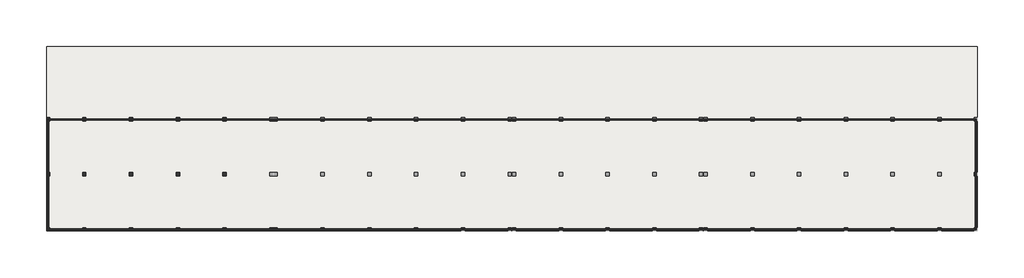
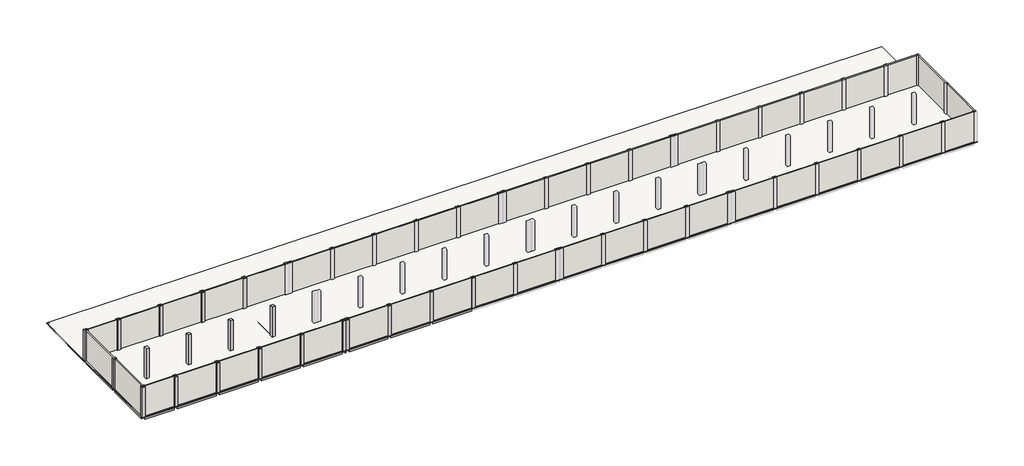
# One storey, part 1 of 4: 38 beams, 20 columns, 4 walls, 2 roofs.
"""IFC4 building model written with IfcOpenShell, lengths in millimetres."""

from ifc_helpers import new_model, si_unit, frame, origin, place, context, project, spatial, polyline, outline, extrude, faceted_brep, element, save

model = new_model("IFC4")

# Units and contexts
model_context = context("Model", 3, world=origin())
ifc_project = project(units=[si_unit("LENGTHUNIT", "METRE", prefix="MILLI")], contexts=[model_context])

# Site, building, storey
site = spatial("IfcSite", under=ifc_project)
building = spatial("IfcBuilding", under=site)
storey = spatial("IfcBuildingStorey", under=building, Name="03_T.O.C_1", Elevation=6949.9618634)

# Beams
placement = place(None, origin())
element("IfcBeam", 1, ObjectType="RC Beam_Rectangular : H_SB_AR_S16_B300xH600", at=placement, inside=storey, context=model_context, shape_type="SweptSolid", body=[
    extrude(outline(polyline([(-4070.0, -6150.4791411), (-4070.0, -5850.4791411), (1630.0, -5850.4791411), (1630.0, -6150.4791411), (-4070.0, -6150.4791411)])), frame((0.0, 0.0, 6349.9618634), z_axis=(0.0, 0.0, 1.0), x_axis=(1.0, 0.0, 0.0)), (0.0, 0.0, 1.0), 499.0),
])
element("IfcBeam", 2, ObjectType="RC Beam_Rectangular : H_SB_AR_S16_B300xH600", at=placement, inside=storey, context=model_context, shape_type="SweptSolid", body=[
    extrude(outline(polyline([(2230.0, -6150.4791411), (2230.0, -5850.4791411), (9830.0, -5850.4791411), (9830.0, -6150.4791411), (2230.0, -6150.4791411)])), frame((0.0, 0.0, 6349.9618634), z_axis=(0.0, 0.0, 1.0), x_axis=(1.0, 0.0, 0.0)), (0.0, 0.0, 1.0), 499.0),
])
element("IfcBeam", 3, ObjectType="RC Beam_Rectangular : H_SB_AR_S16_B300xH600", at=placement, inside=storey, context=model_context, shape_type="SweptSolid", body=[
    extrude(outline(polyline([(10430.0, -6150.4791411), (10430.0, -5850.4791411), (18030.0, -5850.4791411), (18030.0, -6150.4791411), (10430.0, -6150.4791411)])), frame((0.0, 0.0, 6349.9618634), z_axis=(0.0, 0.0, 1.0), x_axis=(1.0, 0.0, 0.0)), (0.0, 0.0, 1.0), 499.0),
])
element("IfcBeam", 4, ObjectType="RC Beam_Rectangular : H_SB_AR_S16_B300xH600", at=placement, inside=storey, context=model_context, shape_type="SweptSolid", body=[
    extrude(outline(polyline([(18630.0, -6150.4791411), (18630.0, -5850.4791411), (26230.0, -5850.4791411), (26230.0, -6150.4791411), (18630.0, -6150.4791411)])), frame((0.0, 0.0, 6349.9618634), z_axis=(0.0, 0.0, 1.0), x_axis=(1.0, 0.0, 0.0)), (0.0, 0.0, 1.0), 499.0),
])
element("IfcBeam", 5, ObjectType="RC Beam_Rectangular : H_SB_AR_S16_B300xH600", at=placement, inside=storey, context=model_context, shape_type="SweptSolid", body=[
    extrude(outline(polyline([(26830.0, -6150.4791411), (26830.0, -5850.4791411), (34430.0, -5850.4791411), (34430.0, -6150.4791411), (26830.0, -6150.4791411)])), frame((0.0, 0.0, 6349.9618634), z_axis=(0.0, 0.0, 1.0), x_axis=(1.0, 0.0, 0.0)), (0.0, 0.0, 1.0), 499.0),
])
element("IfcBeam", 6, ObjectType="RC Beam_Rectangular : H_SB_AR_S16_B300xH600", at=placement, inside=storey, context=model_context, shape_type="SweptSolid", body=[
    extrude(outline(polyline([(-4070.0, -15800.4791411), (-4070.0, -15500.4791411), (1630.0, -15500.4791411), (1630.0, -15800.4791411), (-4070.0, -15800.4791411)])), frame((0.0, 0.0, 6349.9618634), z_axis=(0.0, 0.0, 1.0), x_axis=(1.0, 0.0, 0.0)), (0.0, 0.0, 1.0), 499.0),
])
element("IfcBeam", 7, ObjectType="RC Beam_Rectangular : H_SB_AR_S16_B300xH600", at=placement, inside=storey, context=model_context, shape_type="SweptSolid", body=[
    extrude(outline(polyline([(2230.0, -15800.4791411), (2230.0, -15500.4791411), (9830.0, -15500.4791411), (9830.0, -15800.4791411), (2230.0, -15800.4791411)])), frame((0.0, 0.0, 6349.9618634), z_axis=(0.0, 0.0, 1.0), x_axis=(1.0, 0.0, 0.0)), (0.0, 0.0, 1.0), 499.0),
])
element("IfcBeam", 8, ObjectType="RC Beam_Rectangular : H_SB_AR_S16_B300xH600", at=placement, inside=storey, context=model_context, shape_type="SweptSolid", body=[
    extrude(outline(polyline([(10430.0, -15800.4791411), (10430.0, -15500.4791411), (18030.0, -15500.4791411), (18030.0, -15800.4791411), (10430.0, -15800.4791411)])), frame((0.0, 0.0, 6349.9618634), z_axis=(0.0, 0.0, 1.0), x_axis=(1.0, 0.0, 0.0)), (0.0, 0.0, 1.0), 499.0),
])
element("IfcBeam", 9, ObjectType="RC Beam_Rectangular : H_SB_AR_S16_B300xH600", at=placement, inside=storey, context=model_context, shape_type="SweptSolid", body=[
    extrude(outline(polyline([(18630.0, -15800.4791411), (18630.0, -15500.4791411), (26230.0, -15500.4791411), (26230.0, -15800.4791411), (18630.0, -15800.4791411)])), frame((0.0, 0.0, 6349.9618634), z_axis=(0.0, 0.0, 1.0), x_axis=(1.0, 0.0, 0.0)), (0.0, 0.0, 1.0), 499.0),
])
element("IfcBeam", 10, ObjectType="RC Beam_Rectangular : H_SB_AR_S16_B300xH600", at=placement, inside=storey, context=model_context, shape_type="SweptSolid", body=[
    extrude(outline(polyline([(26830.0, -15800.4791411), (26830.0, -15500.4791411), (34430.0, -15500.4791411), (34430.0, -15800.4791411), (26830.0, -15800.4791411)])), frame((0.0, 0.0, 6349.9618634), z_axis=(0.0, 0.0, 1.0), x_axis=(1.0, 0.0, 0.0)), (0.0, 0.0, 1.0), 499.0),
])
element("IfcBeam", 11, ObjectType="RC Beam_Rectangular : H_SB_AR_S16_B300xH600", at=placement, inside=storey, context=model_context, shape_type="SweptSolid", body=[
    extrude(outline(polyline([(-4070.0, -25450.4791411), (-4070.0, -25150.4791411), (1630.0, -25150.4791411), (1630.0, -25450.4791411), (-4070.0, -25450.4791411)])), frame((0.0, 0.0, 6349.9618634), z_axis=(0.0, 0.0, 1.0), x_axis=(1.0, 0.0, 0.0)), (0.0, 0.0, 1.0), 499.0),
])
element("IfcBeam", 12, ObjectType="RC Beam_Rectangular : H_SB_AR_S16_B300xH600", at=placement, inside=storey, context=model_context, shape_type="SweptSolid", body=[
    extrude(outline(polyline([(2230.0, -25450.4791411), (2230.0, -25150.4791411), (9830.0, -25150.4791411), (9830.0, -25450.4791411), (2230.0, -25450.4791411)])), frame((0.0, 0.0, 6349.9618634), z_axis=(0.0, 0.0, 1.0), x_axis=(1.0, 0.0, 0.0)), (0.0, 0.0, 1.0), 499.0),
])
element("IfcBeam", 13, ObjectType="RC Beam_Rectangular : H_SB_AR_S16_B300xH600", at=placement, inside=storey, context=model_context, shape_type="SweptSolid", body=[
    extrude(outline(polyline([(10430.0, -25450.4791411), (10430.0, -25150.4791411), (18030.0, -25150.4791411), (18030.0, -25450.4791411), (10430.0, -25450.4791411)])), frame((0.0, 0.0, 6349.9618634), z_axis=(0.0, 0.0, 1.0), x_axis=(1.0, 0.0, 0.0)), (0.0, 0.0, 1.0), 499.0),
])
element("IfcBeam", 14, ObjectType="RC Beam_Rectangular : H_SB_AR_S16_B300xH600", at=placement, inside=storey, context=model_context, shape_type="SweptSolid", body=[
    extrude(outline(polyline([(18630.0, -25450.4791411), (18630.0, -25150.4791411), (26230.0, -25150.4791411), (26230.0, -25450.4791411), (18630.0, -25450.4791411)])), frame((0.0, 0.0, 6349.9618634), z_axis=(0.0, 0.0, 1.0), x_axis=(1.0, 0.0, 0.0)), (0.0, 0.0, 1.0), 499.0),
])
element("IfcBeam", 15, ObjectType="RC Beam_Rectangular : H_SB_AR_S16_B300xH600", at=placement, inside=storey, context=model_context, shape_type="SweptSolid", body=[
    extrude(outline(polyline([(26830.0, -25450.4791411), (26830.0, -25150.4791411), (34430.0, -25150.4791411), (34430.0, -25450.4791411), (26830.0, -25450.4791411)])), frame((0.0, 0.0, 6349.9618634), z_axis=(0.0, 0.0, 1.0), x_axis=(1.0, 0.0, 0.0)), (0.0, 0.0, 1.0), 499.0),
])
element("IfcBeam", 16, ObjectType="RC Beam_Rectangular : H_SB_AR_S16_B300xH600", at=placement, inside=storey, context=model_context, shape_type="SweptSolid", body=[
    extrude(outline(polyline([(35030.0, -25450.4791411), (35030.0, -25150.4791411), (35180.0, -25150.4791411), (35180.0, -25450.4791411), (35030.0, -25450.4791411)])), frame((0.0, 0.0, 6349.9618634), z_axis=(0.0, 0.0, 1.0), x_axis=(1.0, 0.0, 0.0)), (0.0, 0.0, 1.0), 499.0),
])
element("IfcBeam", 17, ObjectType="RC Beam_Rectangular : H_SB_AR_S16_B300xH600", at=placement, inside=storey, context=model_context, shape_type="SweptSolid", body=[
    extrude(outline(polyline([(35780.0, -25450.4791411), (35780.0, -25150.4791411), (43380.0, -25150.4791411), (43380.0, -25450.4791411), (35780.0, -25450.4791411)])), frame((0.0, 0.0, 6349.9618634), z_axis=(0.0, 0.0, 1.0), x_axis=(1.0, 0.0, 0.0)), (0.0, 0.0, 1.0), 499.0),
])
element("IfcBeam", 18, ObjectType="RC Beam_Rectangular : H_SB_AR_S16_B300xH600", at=placement, inside=storey, context=model_context, shape_type="SweptSolid", body=[
    extrude(outline(polyline([(43980.0, -25450.4791411), (43980.0, -25150.4791411), (51580.0, -25150.4791411), (51580.0, -25450.4791411), (43980.0, -25450.4791411)])), frame((0.0, 0.0, 6349.9618634), z_axis=(0.0, 0.0, 1.0), x_axis=(1.0, 0.0, 0.0)), (0.0, 0.0, 1.0), 499.0),
])
element("IfcBeam", 19, ObjectType="RC Beam_Rectangular : H_SB_AR_S16_B300xH600", at=placement, inside=storey, context=model_context, shape_type="SweptSolid", body=[
    extrude(outline(polyline([(52180.0, -25450.4791411), (52180.0, -25150.4791411), (59780.0, -25150.4791411), (59780.0, -25450.4791411), (52180.0, -25450.4791411)])), frame((0.0, 0.0, 6349.9618634), z_axis=(0.0, 0.0, 1.0), x_axis=(1.0, 0.0, 0.0)), (0.0, 0.0, 1.0), 499.0),
])
element("IfcBeam", 20, ObjectType="RC Beam_Rectangular : H_SB_AR_S16_B300xH600", at=placement, inside=storey, context=model_context, shape_type="SweptSolid", body=[
    extrude(outline(polyline([(-4520.0, -15950.4791411), (-4220.0, -15950.4791411), (-4220.0, -25000.4791411), (-4520.0, -25000.4791411), (-4520.0, -15950.4791411)])), frame((0.0, 0.0, 6349.9618634), z_axis=(0.0, 0.0, 1.0), x_axis=(1.0, 0.0, 0.0)), (0.0, 0.0, 1.0), 499.0),
])
element("IfcBeam", 21, ObjectType="RC Beam_Rectangular : H_SB_AR_S16_B300xH600", at=placement, inside=storey, context=model_context, shape_type="SweptSolid", body=[
    extrude(outline(polyline([(-4520.0, -6300.4791411), (-4220.0, -6300.4791411), (-4220.0, -15350.4791411), (-4520.0, -15350.4791411), (-4520.0, -6300.4791411)])), frame((0.0, 0.0, 6349.9618634), z_axis=(0.0, 0.0, 1.0), x_axis=(1.0, 0.0, 0.0)), (0.0, 0.0, 1.0), 499.0),
])
element("IfcBeam", 22, ObjectType="RC Beam_Rectangular : H_SB_AR_S16_B300xH600", at=placement, inside=storey, context=model_context, shape_type="SweptSolid", body=[
    extrude(outline(polyline([(-4520.0, -50.4791411), (-4220.0, -50.4791411), (-4220.0, -5700.4791411), (-4520.0, -5700.4791411), (-4520.0, -50.4791411)])), frame((0.0, 0.0, 6349.9618634), z_axis=(0.0, 0.0, 1.0), x_axis=(1.0, 0.0, 0.0)), (0.0, 0.0, 1.0), 499.0),
])
element("IfcBeam", 23, ObjectType="RC Beam_Rectangular : H_SB_AR_S16_B300xH600", at=placement, inside=storey, context=model_context, shape_type="SweptSolid", body=[
    extrude(outline(polyline([(1780.0, -15950.4791411), (2080.0, -15950.4791411), (2080.0, -25000.4791411), (1780.0, -25000.4791411), (1780.0, -15950.4791411)])), frame((0.0, 0.0, 6349.9618634), z_axis=(0.0, 0.0, 1.0), x_axis=(1.0, 0.0, 0.0)), (0.0, 0.0, 1.0), 499.0),
])
element("IfcBeam", 24, ObjectType="RC Beam_Rectangular : H_SB_AR_S16_B300xH600", at=placement, inside=storey, context=model_context, shape_type="SweptSolid", body=[
    extrude(outline(polyline([(1780.0, -6300.4791411), (2080.0, -6300.4791411), (2080.0, -15350.4791411), (1780.0, -15350.4791411), (1780.0, -6300.4791411)])), frame((0.0, 0.0, 6349.9618634), z_axis=(0.0, 0.0, 1.0), x_axis=(1.0, 0.0, 0.0)), (0.0, 0.0, 1.0), 499.0),
])
element("IfcBeam", 25, ObjectType="RC Beam_Rectangular : H_SB_AR_S16_B300xH600", at=placement, inside=storey, context=model_context, shape_type="SweptSolid", body=[
    extrude(outline(polyline([(1780.0, 99.5208589), (2080.0, 99.5208589), (2080.0, -5700.4791411), (1780.0, -5700.4791411), (1780.0, 99.5208589)])), frame((0.0, 0.0, 6349.9618634), z_axis=(0.0, 0.0, 1.0), x_axis=(1.0, 0.0, 0.0)), (0.0, 0.0, 1.0), 499.0),
])
element("IfcBeam", 26, ObjectType="RC Beam_Rectangular : H_SB_AR_S16_B300xH600", at=placement, inside=storey, context=model_context, shape_type="SweptSolid", body=[
    extrude(outline(polyline([(9980.0, -15950.4791411), (10280.0, -15950.4791411), (10280.0, -25000.4791411), (9980.0, -25000.4791411), (9980.0, -15950.4791411)])), frame((0.0, 0.0, 6349.9618634), z_axis=(0.0, 0.0, 1.0), x_axis=(1.0, 0.0, 0.0)), (0.0, 0.0, 1.0), 499.0),
])
element("IfcBeam", 27, ObjectType="RC Beam_Rectangular : H_SB_AR_S16_B300xH600", at=placement, inside=storey, context=model_context, shape_type="SweptSolid", body=[
    extrude(outline(polyline([(9980.0, -6300.4791411), (10280.0, -6300.4791411), (10280.0, -15350.4791411), (9980.0, -15350.4791411), (9980.0, -6300.4791411)])), frame((0.0, 0.0, 6349.9618634), z_axis=(0.0, 0.0, 1.0), x_axis=(1.0, 0.0, 0.0)), (0.0, 0.0, 1.0), 499.0),
])
element("IfcBeam", 28, ObjectType="RC Beam_Rectangular : H_SB_AR_S16_B300xH600", at=placement, inside=storey, context=model_context, shape_type="SweptSolid", body=[
    extrude(outline(polyline([(9980.0, 99.5208589), (10280.0, 99.5208589), (10280.0, -5700.4791411), (9980.0, -5700.4791411), (9980.0, 99.5208589)])), frame((0.0, 0.0, 6349.9618634), z_axis=(0.0, 0.0, 1.0), x_axis=(1.0, 0.0, 0.0)), (0.0, 0.0, 1.0), 499.0),
])
element("IfcBeam", 29, ObjectType="RC Beam_Rectangular : H_SB_AR_S16_B300xH600", at=placement, inside=storey, context=model_context, shape_type="SweptSolid", body=[
    extrude(outline(polyline([(18180.0, -15950.4791411), (18480.0, -15950.4791411), (18480.0, -25000.4791411), (18180.0, -25000.4791411), (18180.0, -15950.4791411)])), frame((0.0, 0.0, 6349.9618634), z_axis=(0.0, 0.0, 1.0), x_axis=(1.0, 0.0, 0.0)), (0.0, 0.0, 1.0), 499.0),
])
element("IfcBeam", 30, ObjectType="RC Beam_Rectangular : H_SB_AR_S16_B300xH600", at=placement, inside=storey, context=model_context, shape_type="SweptSolid", body=[
    extrude(outline(polyline([(18180.0, -6300.4791411), (18480.0, -6300.4791411), (18480.0, -15350.4791411), (18180.0, -15350.4791411), (18180.0, -6300.4791411)])), frame((0.0, 0.0, 6349.9618634), z_axis=(0.0, 0.0, 1.0), x_axis=(1.0, 0.0, 0.0)), (0.0, 0.0, 1.0), 499.0),
])
element("IfcBeam", 31, ObjectType="RC Beam_Rectangular : H_SB_AR_S16_B300xH600", at=placement, inside=storey, context=model_context, shape_type="SweptSolid", body=[
    extrude(outline(polyline([(18180.0, 99.5208589), (18480.0, 99.5208589), (18480.0, -5700.4791411), (18180.0, -5700.4791411), (18180.0, 99.5208589)])), frame((0.0, 0.0, 6349.9618634), z_axis=(0.0, 0.0, 1.0), x_axis=(1.0, 0.0, 0.0)), (0.0, 0.0, 1.0), 499.0),
])
element("IfcBeam", 32, ObjectType="RC Beam_Rectangular : H_SB_AR_S16_B300xH600", at=placement, inside=storey, context=model_context, shape_type="SweptSolid", body=[
    extrude(outline(polyline([(26380.0, -15950.4791411), (26680.0, -15950.4791411), (26680.0, -25000.4791411), (26380.0, -25000.4791411), (26380.0, -15950.4791411)])), frame((0.0, 0.0, 6349.9618634), z_axis=(0.0, 0.0, 1.0), x_axis=(1.0, 0.0, 0.0)), (0.0, 0.0, 1.0), 499.0),
])
element("IfcBeam", 33, ObjectType="RC Beam_Rectangular : H_SB_AR_S16_B300xH600", at=placement, inside=storey, context=model_context, shape_type="SweptSolid", body=[
    extrude(outline(polyline([(26380.0, -6300.4791411), (26680.0, -6300.4791411), (26680.0, -15350.4791411), (26380.0, -15350.4791411), (26380.0, -6300.4791411)])), frame((0.0, 0.0, 6349.9618634), z_axis=(0.0, 0.0, 1.0), x_axis=(1.0, 0.0, 0.0)), (0.0, 0.0, 1.0), 499.0),
])
element("IfcBeam", 34, ObjectType="RC Beam_Rectangular : H_SB_AR_S16_B300xH600", at=placement, inside=storey, context=model_context, shape_type="SweptSolid", body=[
    extrude(outline(polyline([(26380.0, 99.5208589), (26680.0, 99.5208589), (26680.0, -5700.4791411), (26380.0, -5700.4791411), (26380.0, 99.5208589)])), frame((0.0, 0.0, 6349.9618634), z_axis=(0.0, 0.0, 1.0), x_axis=(1.0, 0.0, 0.0)), (0.0, 0.0, 1.0), 499.0),
])
element("IfcBeam", 35, ObjectType="RC Beam_Rectangular : H_SB_AR_S16_B300xH600", at=placement, inside=storey, context=model_context, shape_type="SweptSolid", body=[
    extrude(outline(polyline([(34580.0, -15950.4791411), (34880.0, -15950.4791411), (34880.0, -25000.4791411), (34580.0, -25000.4791411), (34580.0, -15950.4791411)])), frame((0.0, 0.0, 6349.9618634), z_axis=(0.0, 0.0, 1.0), x_axis=(1.0, 0.0, 0.0)), (0.0, 0.0, 1.0), 499.0),
])
element("IfcBeam", 36, ObjectType="RC Beam_Rectangular : H_SB_AR_S16_B300xH600", at=placement, inside=storey, context=model_context, shape_type="SweptSolid", body=[
    extrude(outline(polyline([(35330.0, -15950.4791411), (35630.0, -15950.4791411), (35630.0, -25000.4791411), (35330.0, -25000.4791411), (35330.0, -15950.4791411)])), frame((0.0, 0.0, 6349.9618634), z_axis=(0.0, 0.0, 1.0), x_axis=(1.0, 0.0, 0.0)), (0.0, 0.0, 1.0), 499.0),
])
element("IfcBeam", 37, ObjectType="RC Beam_Rectangular : H_SB_AR_S16_B300xH600", at=placement, inside=storey, context=model_context, shape_type="SweptSolid", body=[
    extrude(outline(polyline([(43530.0, -15950.4791411), (43830.0, -15950.4791411), (43830.0, -25000.4791411), (43530.0, -25000.4791411), (43530.0, -15950.4791411)])), frame((0.0, 0.0, 6349.9618634), z_axis=(0.0, 0.0, 1.0), x_axis=(1.0, 0.0, 0.0)), (0.0, 0.0, 1.0), 499.0),
])
element("IfcBeam", 38, ObjectType="RC Beam_Rectangular : H_SB_AR_S16_B300xH600", at=placement, inside=storey, context=model_context, shape_type="SweptSolid", body=[
    extrude(outline(polyline([(51730.0, -15950.4791411), (52030.0, -15950.4791411), (52030.0, -25000.4791411), (51730.0, -25000.4791411), (51730.0, -15950.4791411)])), frame((0.0, 0.0, 6349.9618634), z_axis=(0.0, 0.0, 1.0), x_axis=(1.0, 0.0, 0.0)), (0.0, 0.0, 1.0), 499.0),
])

# Columns
element("IfcColumn", 39, ObjectType="RC_Column_Rectangular : H_SC_AR_S15_W600xL600", at=placement, inside=storey, context=model_context, shape_type="SweptSolid", body=[
    extrude(outline(polyline([(-4070.0, -5700.4791411), (-4070.0, -6300.4791411), (-4670.0, -6300.4791411), (-4670.0, -5700.4791411), (-4070.0, -5700.4791411)])), frame((0.0, 0.0, 6949.9618634), z_axis=(0.0, 0.0, 1.0), x_axis=(1.0, 0.0, 0.0)), (0.0, 0.0, 1.0), 6200.0),
])
element("IfcColumn", 40, ObjectType="RC_Column_Rectangular : H_SC_AR_S15_W600xL600", at=placement, inside=storey, context=model_context, shape_type="SweptSolid", body=[
    extrude(outline(polyline([(2230.0, -5700.4791411), (2230.0, -6300.4791411), (1630.0, -6300.4791411), (1630.0, -5700.4791411), (2230.0, -5700.4791411)])), frame((0.0, 0.0, 6949.9618634), z_axis=(0.0, 0.0, 1.0), x_axis=(1.0, 0.0, 0.0)), (0.0, 0.0, 1.0), 6200.0),
])
element("IfcColumn", 41, ObjectType="RC_Column_Rectangular : H_SC_AR_S15_W600xL600", at=placement, inside=storey, context=model_context, shape_type="SweptSolid", body=[
    extrude(outline(polyline([(10430.0, -5700.4791411), (10430.0, -6300.4791411), (9830.0, -6300.4791411), (9830.0, -5700.4791411), (10430.0, -5700.4791411)])), frame((0.0, 0.0, 6949.9618634), z_axis=(0.0, 0.0, 1.0), x_axis=(1.0, 0.0, 0.0)), (0.0, 0.0, 1.0), 6200.0),
])
element("IfcColumn", 42, ObjectType="RC_Column_Rectangular : H_SC_AR_S15_W600xL600", at=placement, inside=storey, context=model_context, shape_type="SweptSolid", body=[
    extrude(outline(polyline([(18630.0, -5700.4791411), (18630.0, -6300.4791411), (18030.0, -6300.4791411), (18030.0, -5700.4791411), (18630.0, -5700.4791411)])), frame((0.0, 0.0, 6949.9618634), z_axis=(0.0, 0.0, 1.0), x_axis=(1.0, 0.0, 0.0)), (0.0, 0.0, 1.0), 6200.0),
])
element("IfcColumn", 43, ObjectType="RC_Column_Rectangular : H_SC_AR_S15_W600xL600", at=placement, inside=storey, context=model_context, shape_type="SweptSolid", body=[
    extrude(outline(polyline([(26830.0, -5700.4791411), (26830.0, -6300.4791411), (26230.0, -6300.4791411), (26230.0, -5700.4791411), (26830.0, -5700.4791411)])), frame((0.0, 0.0, 6949.9618634), z_axis=(0.0, 0.0, 1.0), x_axis=(1.0, 0.0, 0.0)), (0.0, 0.0, 1.0), 6200.0),
])
element("IfcColumn", 44, ObjectType="RC_Column_Rectangular : H_SC_AR_S15_W600xL600", at=placement, inside=storey, context=model_context, shape_type="SweptSolid", body=[
    extrude(outline(polyline([(-4070.0, -15350.4791411), (-4070.0, -15950.4791411), (-4670.0, -15950.4791411), (-4670.0, -15350.4791411), (-4070.0, -15350.4791411)])), frame((0.0, 0.0, 6949.9618634), z_axis=(0.0, 0.0, 1.0), x_axis=(1.0, 0.0, 0.0)), (0.0, 0.0, 1.0), 6200.0),
])
element("IfcColumn", 45, ObjectType="RC_Column_Rectangular : H_SC_AR_S15_W600xL600", at=placement, inside=storey, context=model_context, shape_type="SweptSolid", body=[
    extrude(outline(polyline([(2230.0, -15350.4791411), (2230.0, -15950.4791411), (1630.0, -15950.4791411), (1630.0, -15350.4791411), (2230.0, -15350.4791411)])), frame((0.0, 0.0, 6949.9618634), z_axis=(0.0, 0.0, 1.0), x_axis=(1.0, 0.0, 0.0)), (0.0, 0.0, 1.0), 6200.0),
])
element("IfcColumn", 46, ObjectType="RC_Column_Rectangular : H_SC_AR_S15_W600xL600", at=placement, inside=storey, context=model_context, shape_type="SweptSolid", body=[
    extrude(outline(polyline([(10430.0, -15350.4791411), (10430.0, -15950.4791411), (9830.0, -15950.4791411), (9830.0, -15350.4791411), (10430.0, -15350.4791411)])), frame((0.0, 0.0, 6949.9618634), z_axis=(0.0, 0.0, 1.0), x_axis=(1.0, 0.0, 0.0)), (0.0, 0.0, 1.0), 6200.0),
])
element("IfcColumn", 47, ObjectType="RC_Column_Rectangular : H_SC_AR_S15_W600xL600", at=placement, inside=storey, context=model_context, shape_type="SweptSolid", body=[
    extrude(outline(polyline([(18630.0, -15350.4791411), (18630.0, -15950.4791411), (18030.0, -15950.4791411), (18030.0, -15350.4791411), (18630.0, -15350.4791411)])), frame((0.0, 0.0, 6949.9618634), z_axis=(0.0, 0.0, 1.0), x_axis=(1.0, 0.0, 0.0)), (0.0, 0.0, 1.0), 6200.0),
])
element("IfcColumn", 48, ObjectType="RC_Column_Rectangular : H_SC_AR_S15_W600xL600", at=placement, inside=storey, context=model_context, shape_type="SweptSolid", body=[
    extrude(outline(polyline([(26830.0, -15350.4791411), (26830.0, -15950.4791411), (26230.0, -15950.4791411), (26230.0, -15350.4791411), (26830.0, -15350.4791411)])), frame((0.0, 0.0, 6949.9618634), z_axis=(0.0, 0.0, 1.0), x_axis=(1.0, 0.0, 0.0)), (0.0, 0.0, 1.0), 6200.0),
])
element("IfcColumn", 49, ObjectType="RC_Column_Rectangular : H_SC_AR_S15_W600xL600", at=placement, inside=storey, context=model_context, shape_type="SweptSolid", body=[
    extrude(outline(polyline([(-4070.0, -25000.4791411), (-4070.0, -25600.4791411), (-4670.0, -25600.4791411), (-4670.0, -25000.4791411), (-4070.0, -25000.4791411)])), frame((0.0, 0.0, 6949.9618634), z_axis=(0.0, 0.0, 1.0), x_axis=(1.0, 0.0, 0.0)), (0.0, 0.0, 1.0), 6200.0),
])
element("IfcColumn", 50, ObjectType="RC_Column_Rectangular : H_SC_AR_S15_W600xL600", at=placement, inside=storey, context=model_context, shape_type="SweptSolid", body=[
    extrude(outline(polyline([(2230.0, -25000.4791411), (2230.0, -25600.4791411), (1630.0, -25600.4791411), (1630.0, -25000.4791411), (2230.0, -25000.4791411)])), frame((0.0, 0.0, 6949.9618634), z_axis=(0.0, 0.0, 1.0), x_axis=(1.0, 0.0, 0.0)), (0.0, 0.0, 1.0), 6200.0),
])
element("IfcColumn", 51, ObjectType="RC_Column_Rectangular : H_SC_AR_S15_W600xL600", at=placement, inside=storey, context=model_context, shape_type="SweptSolid", body=[
    extrude(outline(polyline([(10430.0, -25000.4791411), (10430.0, -25600.4791411), (9830.0, -25600.4791411), (9830.0, -25000.4791411), (10430.0, -25000.4791411)])), frame((0.0, 0.0, 6949.9618634), z_axis=(0.0, 0.0, 1.0), x_axis=(1.0, 0.0, 0.0)), (0.0, 0.0, 1.0), 6200.0),
])
element("IfcColumn", 52, ObjectType="RC_Column_Rectangular : H_SC_AR_S15_W600xL600", at=placement, inside=storey, context=model_context, shape_type="SweptSolid", body=[
    extrude(outline(polyline([(18630.0, -25000.4791411), (18630.0, -25600.4791411), (18030.0, -25600.4791411), (18030.0, -25000.4791411), (18630.0, -25000.4791411)])), frame((0.0, 0.0, 6949.9618634), z_axis=(0.0, 0.0, 1.0), x_axis=(1.0, 0.0, 0.0)), (0.0, 0.0, 1.0), 6200.0),
])
element("IfcColumn", 53, ObjectType="RC_Column_Rectangular : H_SC_AR_S15_W600xL600", at=placement, inside=storey, context=model_context, shape_type="SweptSolid", body=[
    extrude(outline(polyline([(26830.0, -25000.4791411), (26830.0, -25600.4791411), (26230.0, -25600.4791411), (26230.0, -25000.4791411), (26830.0, -25000.4791411)])), frame((0.0, 0.0, 6949.9618634), z_axis=(0.0, 0.0, 1.0), x_axis=(1.0, 0.0, 0.0)), (0.0, 0.0, 1.0), 6200.0),
])
element("IfcColumn", 54, ObjectType="RC_Column_Rectangular : H_SC_AR_S15_W600xL600", at=placement, inside=storey, context=model_context, shape_type="SweptSolid", body=[
    extrude(outline(polyline([(35030.0, -25000.4791411), (35030.0, -25600.4791411), (34430.0, -25600.4791411), (34430.0, -25000.4791411), (35030.0, -25000.4791411)])), frame((0.0, 0.0, 6949.9618634), z_axis=(0.0, 0.0, 1.0), x_axis=(1.0, 0.0, 0.0)), (0.0, 0.0, 1.0), 6200.0),
])
element("IfcColumn", 55, ObjectType="RC_Column_Rectangular : H_SC_AR_S15_W600xL600", at=placement, inside=storey, context=model_context, shape_type="SweptSolid", body=[
    extrude(outline(polyline([(35780.0, -25000.4791411), (35780.0, -25600.4791411), (35180.0, -25600.4791411), (35180.0, -25000.4791411), (35780.0, -25000.4791411)])), frame((0.0, 0.0, 6949.9618634), z_axis=(0.0, 0.0, 1.0), x_axis=(1.0, 0.0, 0.0)), (0.0, 0.0, 1.0), 6200.0),
])
element("IfcColumn", 56, ObjectType="RC_Column_Rectangular : H_SC_AR_S15_W600xL600", at=placement, inside=storey, context=model_context, shape_type="SweptSolid", body=[
    extrude(outline(polyline([(43980.0, -25000.4791411), (43980.0, -25600.4791411), (43380.0, -25600.4791411), (43380.0, -25000.4791411), (43980.0, -25000.4791411)])), frame((0.0, 0.0, 6949.9618634), z_axis=(0.0, 0.0, 1.0), x_axis=(1.0, 0.0, 0.0)), (0.0, 0.0, 1.0), 6200.0),
])
element("IfcColumn", 57, ObjectType="RC_Column_Rectangular : H_SC_AR_S15_W600xL600", at=placement, inside=storey, context=model_context, shape_type="SweptSolid", body=[
    extrude(outline(polyline([(52180.0, -25000.4791411), (52180.0, -25600.4791411), (51580.0, -25600.4791411), (51580.0, -25000.4791411), (52180.0, -25000.4791411)])), frame((0.0, 0.0, 6949.9618634), z_axis=(0.0, 0.0, 1.0), x_axis=(1.0, 0.0, 0.0)), (0.0, 0.0, 1.0), 6200.0),
])
element("IfcColumn", 58, ObjectType="RC_Column_Rectangular : H_SC_AR_S15_W600xL600", at=placement, inside=storey, context=model_context, shape_type="SweptSolid", body=[
    extrude(outline(polyline([(60380.0, -25000.4791411), (60380.0, -25600.4791411), (59780.0, -25600.4791411), (59780.0, -25000.4791411), (60380.0, -25000.4791411)])), frame((0.0, 0.0, 6949.9618634), z_axis=(0.0, 0.0, 1.0), x_axis=(1.0, 0.0, 0.0)), (0.0, 0.0, 1.0), 6200.0),
])

# Roofs
element("IfcRoof", 59, ObjectType="H_RF_AR_B06_Memb_XPS_PE_Protective Conc", at=placement, inside=storey, context=model_context, shape_type="Brep", body=[
    faceted_brep([(158430.0, 6799.5208589, 6848.9618634), (158430.0, 6199.5208589, 6848.9618634), (158430.0, 549.5208589, 6848.9618634), (158430.0, -50.4791411, 6848.9618634), (158430.0, -5700.4791411, 6848.9618634), (158430.0, -6300.4791411, 6848.9618634), (158430.0, -15350.4791411, 6848.9618634), (158430.0, -15950.4791411, 6848.9618634), (158430.0, -25000.4791411, 6848.9618634), (158430.0, -25600.4791411, 6848.9618634), (157830.0, -25600.4791411, 6848.9618634), (152080.0, -25600.4791411, 6848.9618634), (151480.0, -25600.4791411, 6848.9618634), (143880.0, -25600.4791411, 6848.9618634), (143280.0, -25600.4791411, 6848.9618634), (135680.0, -25600.4791411, 6848.9618634), (135080.0, -25600.4791411, 6848.9618634), (127480.0, -25600.4791411, 6848.9618634), (126880.0, -25600.4791411, 6848.9618634), (119280.0, -25600.4791411, 6848.9618634), (118680.0, -25600.4791411, 6848.9618634), (111080.0, -25600.4791411, 6848.9618634), (110480.0, -25600.4791411, 6848.9618634), (110330.0, -25600.4791411, 6848.9618634), (109730.0, -25600.4791411, 6848.9618634), (102130.0, -25600.4791411, 6848.9618634), (101530.0, -25600.4791411, 6848.9618634), (93930.0, -25600.4791411, 6848.9618634), (93330.0, -25600.4791411, 6848.9618634), (85730.0, -25600.4791411, 6848.9618634), (85130.0, -25600.4791411, 6848.9618634), (77530.0, -25600.4791411, 6848.9618634), (76930.0, -25600.4791411, 6848.9618634), (76780.0, -25600.4791411, 6848.9618634), (76180.0, -25600.4791411, 6848.9618634), (68580.0, -25600.4791411, 6848.9618634), (67980.0, -25600.4791411, 6848.9618634), (60380.0, -25600.4791411, 6848.9618634), (59780.0, -25600.4791411, 6848.9618634), (52180.0, -25600.4791411, 6848.9618634), (51580.0, -25600.4791411, 6848.9618634), (43980.0, -25600.4791411, 6848.9618634), (43380.0, -25600.4791411, 6848.9618634), (35780.0, -25600.4791411, 6848.9618634), (35180.0, -25600.4791411, 6848.9618634), (35030.0, -25600.4791411, 6848.9618634), (34430.0, -25600.4791411, 6848.9618634), (26830.0, -25600.4791411, 6848.9618634), (26230.0, -25600.4791411, 6848.9618634), (18630.0, -25600.4791411, 6848.9618634), (18030.0, -25600.4791411, 6848.9618634), (10430.0, -25600.4791411, 6848.9618634), (9830.0, -25600.4791411, 6848.9618634), (2230.0, -25600.4791411, 6848.9618634), (1630.0, -25600.4791411, 6848.9618634), (-4070.0, -25600.4791411, 6848.9618634), (-4670.0, -25600.4791411, 6848.9618634), (-4670.0, -25000.4791411, 6848.9618634), (-4670.0, -15950.4791411, 6848.9618634), (-4670.0, -15350.4791411, 6848.9618634), (-4670.0, -6300.4791411, 6848.9618634), (-4670.0, -5700.4791411, 6848.9618634), (-4670.0, -50.4791411, 6848.9618634), (-4670.0, 549.5208589, 6848.9618634), (-4670.0, 6199.5208589, 6848.9618634), (-4670.0, 6799.5208589, 6848.9618634), (-4070.0, 6799.5208589, 6848.9618634), (1630.0, 6799.5208589, 6848.9618634), (2230.0, 6799.5208589, 6848.9618634), (9830.0, 6799.5208589, 6848.9618634), (10430.0, 6799.5208589, 6848.9618634), (18030.0, 6799.5208589, 6848.9618634), (18630.0, 6799.5208589, 6848.9618634), (26230.0, 6799.5208589, 6848.9618634), (26830.0, 6799.5208589, 6848.9618634), (34430.0, 6799.5208589, 6848.9618634), (35030.0, 6799.5208589, 6848.9618634), (35180.0, 6799.5208589, 6848.9618634), (35780.0, 6799.5208589, 6848.9618634), (43380.0, 6799.5208589, 6848.9618634), (43980.0, 6799.5208589, 6848.9618634), (51580.0, 6799.5208589, 6848.9618634), (52180.0, 6799.5208589, 6848.9618634), (59780.0, 6799.5208589, 6848.9618634), (60380.0, 6799.5208589, 6848.9618634), (67980.0, 6799.5208589, 6848.9618634), (68580.0, 6799.5208589, 6848.9618634), (76180.0, 6799.5208589, 6848.9618634), (76780.0, 6799.5208589, 6848.9618634), (76930.0, 6799.5208589, 6848.9618634), (77530.0, 6799.5208589, 6848.9618634), (85130.0, 6799.5208589, 6848.9618634), (85730.0, 6799.5208589, 6848.9618634), (93330.0, 6799.5208589, 6848.9618634), (93930.0, 6799.5208589, 6848.9618634), (101530.0, 6799.5208589, 6848.9618634), (102130.0, 6799.5208589, 6848.9618634), (109730.0, 6799.5208589, 6848.9618634), (110330.0, 6799.5208589, 6848.9618634), (110480.0, 6799.5208589, 6848.9618634), (111080.0, 6799.5208589, 6848.9618634), (118680.0, 6799.5208589, 6848.9618634), (119280.0, 6799.5208589, 6848.9618634), (126880.0, 6799.5208589, 6848.9618634), (127480.0, 6799.5208589, 6848.9618634), (135080.0, 6799.5208589, 6848.9618634), (135680.0, 6799.5208589, 6848.9618634), (143280.0, 6799.5208589, 6848.9618634), (143880.0, 6799.5208589, 6848.9618634), (151480.0, 6799.5208589, 6848.9618634), (152080.0, 6799.5208589, 6848.9618634), (157830.0, 6799.5208589, 6848.9618634), (158430.0, -25600.4791411, 6949.9618634), (158430.0, 6799.5208589, 6949.9618634), (-4670.0, 6799.5208589, 6949.9618634), (-4670.0, -25600.4791411, 6949.9618634)], [[[0, 1, 2, 3, 4, 5, 6, 7, 8, 9, 10, 11, 12, 13, 14, 15, 16, 17, 18, 19, 20, 21, 22, 23, 24, 25, 26, 27, 28, 29, 30, 31, 32, 33, 34, 35, 36, 37, 38, 39, 40, 41, 42, 43, 44, 45, 46, 47, 48, 49, 50, 51, 52, 53, 54, 55, 56, 57, 58, 59, 60, 61, 62, 63, 64, 65, 66, 67, 68, 69, 70, 71, 72, 73, 74, 75, 76, 77, 78, 79, 80, 81, 82, 83, 84, 85, 86, 87, 88, 89, 90, 91, 92, 93, 94, 95, 96, 97, 98, 99, 100, 101, 102, 103, 104, 105, 106, 107, 108, 109, 110, 111]], [[112, 113, 114, 115]], [[113, 112, 9, 8, 7, 6, 5, 4, 3, 2, 1, 0]], [[114, 113, 0, 111, 110, 109, 108, 107, 106, 105, 104, 103, 102, 101, 100, 99, 98, 97, 96, 95, 94, 93, 92, 91, 90, 89, 88, 87, 86, 85, 84, 83, 82, 81, 80, 79, 78, 77, 76, 75, 74, 73, 72, 71, 70, 69, 68, 67, 66, 65]], [[115, 114, 65, 64, 63, 62, 61, 60, 59, 58, 57, 56]], [[112, 115, 56, 55, 54, 53, 52, 51, 50, 49, 48, 47, 46, 45, 44, 43, 42, 41, 40, 39, 38, 37, 36, 35, 34, 33, 32, 31, 30, 29, 28, 27, 26, 25, 24, 23, 22, 21, 20, 19, 18, 17, 16, 15, 14, 13, 12, 11, 10, 9]]]),
])
element("IfcRoof", 60, ObjectType="H_RF_AR_B06_Memb_XPS_PE_Protective Conc", at=placement, inside=storey, context=model_context, shape_type="SweptSolid", body=[
    extrude(outline(polyline([(-4370.0, 6499.5208589), (158130.0, 6499.5208589), (158130.0, -6000.4791411), (-4370.0, -6000.4791411), (-4370.0, 6499.5208589)])), frame((0.0, 0.0, 6848.9618634), z_axis=(0.0, 0.0, 1.0), x_axis=(1.0, 0.0, 0.0)), (0.0, 0.0, 1.0), 101.0),
])

# Walls
element("IfcWall", 61, ObjectType="H_WA_AR_B02_Ext Wall_RC T200", at=placement, inside=storey, context=model_context, shape_type="Brep", body=[
    faceted_brep([(-4470.0, -6100.4791411, 6949.9618634), (-4270.0, -6100.4791411, 6949.9618634), (158030.0, -6100.4791411, 6949.9618634), (158030.0, -6100.4791411, 13149.9618634), (-4270.0, -6100.4791411, 13149.9618634), (-4470.0, -6100.4791411, 13149.9618634), (-4470.0, -5900.4791411, 6949.9618634), (-4470.0, -5900.4791411, 13149.9618634), (158030.0, -5900.4791411, 13149.9618634), (158030.0, -5900.4791411, 6949.9618634)], [[[0, 1, 2, 3, 4, 5]], [[6, 7, 8, 9]], [[2, 1, 0, 6, 9]], [[5, 4, 3, 8, 7]], [[0, 5, 7, 6]], [[3, 2, 9, 8]]]),
])
element("IfcWall", 62, ObjectType="H_WA_AR_B02_Ext Wall_RC T200", at=placement, inside=storey, context=model_context, shape_type="Brep", body=[
    faceted_brep([(-4270.0, -25400.4791411, 6949.9618634), (-4270.0, -25200.4791411, 6949.9618634), (-4270.0, -6100.4791411, 6949.9618634), (-4270.0, -6100.4791411, 13149.9618634), (-4270.0, -25200.4791411, 13149.9618634), (-4270.0, -25400.4791411, 13149.9618634), (-4470.0, -25400.4791411, 6949.9618634), (-4470.0, -25400.4791411, 13149.9618634), (-4470.0, -6100.4791411, 13149.9618634), (-4470.0, -6100.4791411, 6949.9618634)], [[[0, 1, 2, 3, 4, 5]], [[6, 7, 8, 9]], [[2, 1, 0, 6, 9]], [[5, 4, 3, 8, 7]], [[0, 5, 7, 6]], [[3, 2, 9, 8]]]),
])
element("IfcWall", 63, ObjectType="H_WA_AR_B02_Ext Wall_RC T200", at=placement, inside=storey, context=model_context, shape_type="Brep", body=[
    faceted_brep([(158230.0, -25200.4791411, 6949.9618634), (158030.0, -25200.4791411, 6949.9618634), (-4270.0, -25200.4791411, 6949.9618634), (-4270.0, -25200.4791411, 13149.9618634), (158030.0, -25200.4791411, 13149.9618634), (158230.0, -25200.4791411, 13149.9618634), (158230.0, -25400.4791411, 6949.9618634), (158230.0, -25400.4791411, 13149.9618634), (-4270.0, -25400.4791411, 13149.9618634), (-4270.0, -25400.4791411, 6949.9618634)], [[[0, 1, 2, 3, 4, 5]], [[6, 7, 8, 9]], [[2, 1, 0, 6, 9]], [[5, 4, 3, 8, 7]], [[0, 5, 7, 6]], [[3, 2, 9, 8]]]),
])
element("IfcWall", 64, ObjectType="H_WA_AR_B02_Ext Wall_RC T200", at=placement, inside=storey, context=model_context, shape_type="Brep", body=[
    faceted_brep([(158030.0, -5900.4791411, 6949.9618634), (158030.0, -6100.4791411, 6949.9618634), (158030.0, -25200.4791411, 6949.9618634), (158030.0, -25200.4791411, 13149.9618634), (158030.0, -6100.4791411, 13149.9618634), (158030.0, -5900.4791411, 13149.9618634), (158230.0, -5900.4791411, 6949.9618634), (158230.0, -5900.4791411, 13149.9618634), (158230.0, -25200.4791411, 13149.9618634), (158230.0, -25200.4791411, 6949.9618634)], [[[0, 1, 2, 3, 4, 5]], [[6, 7, 8, 9]], [[2, 1, 0, 6, 9]], [[5, 4, 3, 8, 7]], [[0, 5, 7, 6]], [[3, 2, 9, 8]]]),
])

save(model, "model.ifc")

# Revit data of these elements
# Type "RC Beam_Rectangular : H_SB_AR_S16_B300xH600"
#   중앙부 하부근 = ""
#   중앙부 상부근 = ""
#   중앙부 보조근 = ""
#   중앙부 늑근 = ""
#   외단부 하부근 = ""
#   외단부 상부근 = ""
#   외단부 보조근 = ""
#   외단부 늑근 = ""
#   부호 = "TG3"
#   내단부 하부근 = ""
#   내단부 상부근 = ""
#   내단부 보조근 = ""
#   내단부 늑근 = ""
#   ALL 하부근 = "3-D20"
#   ALL 상부근 = "3-D20"
#   ALL 보조근 = ""
#   ALL 늑근 = "2-D10 @120"
#   Width = 300 mm
#   Height = 600 mm
#   Length [instance default] = 1524 mm
#   b = 300 mm
#   h = 600 mm
#   hec_material3 [instance default] = none
#   hec_material2 [instance default] = none
#   hec_material1 [instance default] = none
#   Structural Material [instance default] = none
#   Assembly Code = ""
# Type "RC_Column_Rectangular : H_SC_AR_S15_W600xL600"
#   Width = 600 mm
#   Length = 600 mm
#   hec_material3 [instance default] = none
#   hec_material2 [instance default] = none
#   hec_material1 [instance default] = none
#   Structural Material [instance default] = none
#   Description = (empty or 0)
# Type "H_RF_AR_B06_Memb_XPS_PE_Protective Conc"
#   Layers, outside or top first: 50 mm no material (function 4); 0 mm no material (function 100); 50 mm no material (function 3); 1 mm no material (function 2)
# Type "H_WA_AR_B02_Ext Wall_RC T200"
#   Type Comments = ""
#   Layers, outside or top first: 0 mm no material (function 100); 0 mm no material (function 100); 200 mm no material (function 1); 0 mm no material (function 100); 0 mm no material (function 100); 0 mm no material (function 100)
# Elements 1, 2, 3, 4, 5, 6, 7, 8, 9, 10, 11, 12, 13, 14, 15, 16, 17, 18, 19, 20, 21, 22, 23, 24, 25, 26, 27, 28, 29, 30, 31, 32, 33, 34, 35, 36, 37, 38 (IfcBeam, "RC Beam_Rectangular : H_SB_AR_S16_B300xH600")
#   Comments = ""
#   hec_material3 = none
#   hec_material2 = none
#   hec_material1 = none
#   Structural Material = none
#   Phase Created = New Construction
# Elements 39, 40, 41, 42, 43, 44, 45, 46, 47, 48, 49, 50, 51, 52, 53, 54, 55, 56, 57, 58 (IfcColumn, "RC_Column_Rectangular : H_SC_AR_S15_W600xL600")
#   Comments = ""
#   hec_material3 = none
#   hec_material2 = none
#   hec_material1 = none
#   Structural Material = none
#   Phase Created = New Construction
# Elements 59, 60 (IfcRoof, "H_RF_AR_B06_Memb_XPS_PE_Protective Conc")
#   built-in parameter 1001705 = 22.8017 (stored number, unit not read)
#   built-in parameter 1001701 = -0.331365 (stored number, unit not read)
#   built-in parameter 1001710 = 33615
#   Phase Created = New Construction
#   Materials on its faces: "Default Roof"
# Elements 61, 62, 63, 64 (IfcWall, "H_WA_AR_B02_Ext Wall_RC T200")
#   Top Offset = 0 mm
#   Base Offset = 0 mm
#   wall height = 6200 mm
#   Phase Created = New Construction
#   Base Constraint = 03_T.O.C_1
#   Top Constraint = 04_T.O.C_2
#   Materials on its faces: "Default Wall"
# Materials
#   "Default Roof": class "Miscellaneous", colour RGB 80 80 80, transparency 0
#   "Default Wall": class "Miscellaneous", colour RGB 80 80 80, transparency 0
